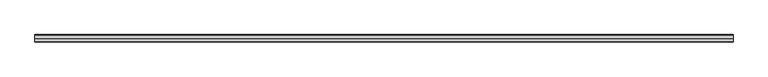
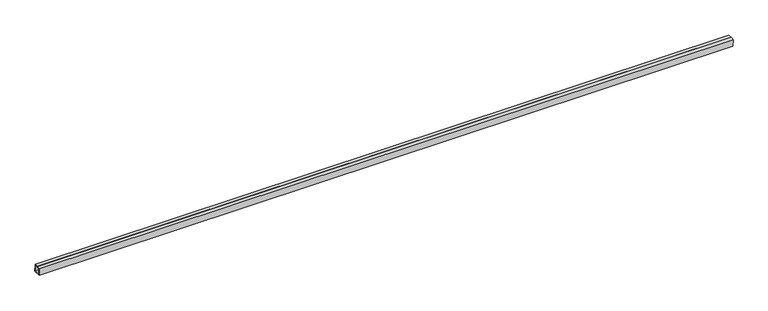
"""IFC4 building model written with IfcOpenShell, lengths in millimetres: proxy geometry, Inner panel:Inner panel:1:Inner panel:1 : Inner panel:Inner panel:300324:2:Inner panel:1:Inner panel:1 : Inner panel:Inner panel:300324:2 : Inner panel:Inner panel:1:Inner panel:1 : Inner panel:Inner panel:300324:300043:23 : Inner panel:Inner panel:1:Inner panel:1 : Inner panel:Inner panel:300324:2:Inner panel:1:Inner panel:1 : Inner panel:Inner panel:300324:2 : Inner panel:Inner panel:1:Inner panel:1 : Inner panel:Inner panel:300324:300043:308120."""

import ifcopenshell
import ifcopenshell.guid

model = None  # the IFC model being written
_history = None  # IfcOwnerHistory: only IFC2X3 demands one
_inside = {}  # id of a spatial element -> (the spatial element, [elements in it])
_under = {}  # id of a project, library or spatial element -> (it, [spatial elements below it])
_declared = {}  # id of a project -> (the project, [libraries it declares])
_typed = {}  # id of a type object -> (the type object, [elements of that type])
_made_of = {}  # id of a material, layer set ... -> (it, [elements and type objects made of it])


def new_model(schema):
    """Start an empty IFC model of exactly this schema.

    Asked for "IFC4X3", IfcOpenShell would pick the latest addendum, in which some entities
    have other attributes; the version numbers below select the first issue.
    IFC2X3 requires an IfcOwnerHistory on every rooted entity: one is made here for all.
    """
    global model, _history
    if schema == "IFC4X3":
        model = ifcopenshell.file(schema_version=(4, 3, 0, 0))
    else:
        model = ifcopenshell.file(schema=schema)
    _inside.clear()
    _under.clear()
    _declared.clear()
    _typed.clear()
    _made_of.clear()
    _history = None
    if model.schema == "IFC2X3":
        org = make("IfcOrganization", Name="unknown")
        user = make(
            "IfcPersonAndOrganization",
            ThePerson=make("IfcPerson", FamilyName="unknown"),
            TheOrganization=org,
        )
        app = make(
            "IfcApplication",
            ApplicationDeveloper=org,
            Version="unknown",
            ApplicationFullName="unknown",
            ApplicationIdentifier="unknown",
        )
        _history = make(
            "IfcOwnerHistory",
            OwningUser=user,
            OwningApplication=app,
            ChangeAction="ADDED",
            CreationDate=0,
        )
    return model


def make(cls, **values):
    """One entity of the class cls with the attributes given. An attribute that is None is left unset."""
    return model.create_entity(
        cls, **{name: value for name, value in values.items() if value is not None}
    )


def rooted(cls, **values):
    """An entity with a GlobalId (a new one), such as an element, a storey or a relation."""
    return make(cls, GlobalId=ifcopenshell.guid.new(), OwnerHistory=_history, **values)


def si_unit(unit_type, name, prefix=None):
    """IfcSIUnit, for example si_unit("LENGTHUNIT", "METRE", prefix="MILLI")."""
    return make("IfcSIUnit", UnitType=unit_type, Prefix=prefix, Name=name)


def assignment(units):
    """IfcUnitAssignment: the units of a project."""
    return None if units is None else make("IfcUnitAssignment", Units=units)


def point(xyz):
    """IfcCartesianPoint."""
    return None if xyz is None else make("IfcCartesianPoint", Coordinates=xyz)


def direction(xyz):
    """IfcDirection."""
    return None if xyz is None else make("IfcDirection", DirectionRatios=xyz)


def frame(location, z_axis=None, x_axis=None):
    """IfcAxis2Placement3D, a coordinate frame: its origin and axes. An axis left out is left unset."""
    return make(
        "IfcAxis2Placement3D",
        Location=point(location),
        Axis=direction(z_axis),
        RefDirection=direction(x_axis),
    )


def origin():
    """The frame at (0, 0, 0) with its axes left unset."""
    return frame((0.0, 0.0, 0.0))


def place(relative_to, where):
    """IfcLocalPlacement: puts the frame where relative to a parent placement (None: the world)."""
    return make(
        "IfcLocalPlacement", PlacementRelTo=relative_to, RelativePlacement=where
    )


def context(
    kind, dimensions, precision=None, world=None, true_north=None, identifier=None
):
    """IfcGeometricRepresentationContext, for example the 3D "Model" context."""
    return make(
        "IfcGeometricRepresentationContext",
        ContextIdentifier=identifier,
        ContextType=kind,
        CoordinateSpaceDimension=dimensions,
        Precision=precision,
        WorldCoordinateSystem=world,
        TrueNorth=true_north,
    )


def project(units=None, contexts=None):
    """IfcProject with its units and contexts."""
    return rooted(
        "IfcProject",
        Name="project",
        RepresentationContexts=contexts,
        UnitsInContext=assignment(units),
    )


def spatial(cls, under=None, at=None, **own):
    """A site, building, storey or space (cls), placed at a placement, below another one or the project."""
    s = rooted(cls, ObjectPlacement=at, **own)
    if under is not None:
        _under.setdefault(under.id(), (under, []))[1].append(s)
    return s


def polyline(points):
    """IfcPolyline through the points."""
    return make("IfcPolyline", Points=[point(p) for p in points])


def outline(outer, holes=None, kind="AREA"):
    """IfcArbitraryClosedProfileDef: a profile drawn as a closed curve; with holes, ...WithVoids."""
    if holes is None:
        return make("IfcArbitraryClosedProfileDef", ProfileType=kind, OuterCurve=outer)
    return make(
        "IfcArbitraryProfileDefWithVoids",
        ProfileType=kind,
        OuterCurve=outer,
        InnerCurves=holes,
    )


def extrude(swept, where, along, depth):
    """IfcExtrudedAreaSolid: the profile swept, set in the frame where, extruded along a direction by depth."""
    return make(
        "IfcExtrudedAreaSolid",
        SweptArea=swept,
        Position=where,
        ExtrudedDirection=direction(along),
        Depth=depth,
    )


def shape(context_of_items, identifier, shape_type, items):
    """IfcShapeRepresentation: the items that make up one representation, for example the "Body"."""
    return make(
        "IfcShapeRepresentation",
        ContextOfItems=context_of_items,
        RepresentationIdentifier=identifier,
        RepresentationType=shape_type,
        Items=items,
    )


def source(mapping_origin, context_of_items, identifier, shape_type, items):
    """IfcRepresentationMap: a shape defined once, which mapped items show again and again."""
    return make(
        "IfcRepresentationMap",
        MappingOrigin=mapping_origin,
        MappedRepresentation=shape(context_of_items, identifier, shape_type, items),
    )


def transform(
    local_origin,
    x_axis=None,
    y_axis=None,
    z_axis=None,
    scale=None,
    scale2=None,
    scale3=None,
    uniform=True,
):
    """IfcCartesianTransformationOperator3D, or its non-uniform kind. x_axis, y_axis, z_axis: its Axis1, 2, 3."""
    if uniform:
        return make(
            "IfcCartesianTransformationOperator3D",
            Axis1=direction(x_axis),
            Axis2=direction(y_axis),
            LocalOrigin=point(local_origin),
            Scale=scale,
            Axis3=direction(z_axis),
        )
    return make(
        "IfcCartesianTransformationOperator3DnonUniform",
        Axis1=direction(x_axis),
        Axis2=direction(y_axis),
        LocalOrigin=point(local_origin),
        Scale=scale,
        Axis3=direction(z_axis),
        Scale2=scale2,
        Scale3=scale3,
    )


def mapped(mapping_source, mapping_target):
    """IfcMappedItem: shows the shape of a source again, moved by a transform."""
    return make(
        "IfcMappedItem", MappingSource=mapping_source, MappingTarget=mapping_target
    )


def made_of(thing, what):
    """Note that an element or type object is made of a material, layer set ...; save() writes the relation."""
    if what is not None:
        _made_of.setdefault(what.id(), (what, []))[1].append(thing)
    return thing


def element(
    cls,
    number,
    at=None,
    inside=None,
    cuts=None,
    type_object=None,
    material=None,
    context=None,
    identifier="Body",
    shape_type=None,
    held_by="IfcProductDefinitionShape",
    body=None,
    shapes=None,
    **own,
):
    """One element of the class cls, such as IfcWall. Its Tag is "e" and its number.

    at: its placement. inside: the storey or other place that contains it. cuts: it is an
    opening in that element (IfcRelVoidsElement). A single representation is given by context,
    identifier, shape_type and body (its items); several are given by shapes. held_by: the class
    of the entity that holds the representations. save() writes the other relations.
    """
    e = rooted(cls, Tag="e%d" % number, ObjectPlacement=at, **own)
    if body is not None:
        shapes = [shape(context, identifier, shape_type, body)]
    if shapes is not None:
        e.Representation = make(held_by, Representations=shapes)
    if inside is not None:
        _inside.setdefault(inside.id(), (inside, []))[1].append(e)
    if cuts is not None:
        rooted(
            "IfcRelVoidsElement", RelatingBuildingElement=cuts, RelatedOpeningElement=e
        )
    if type_object is not None:
        _typed.setdefault(type_object.id(), (type_object, []))[1].append(e)
    return made_of(e, material)


def aggregate(whole, parts):
    """IfcRelAggregates: a whole, such as a stair, and the parts it consists of."""
    return rooted("IfcRelAggregates", RelatingObject=whole, RelatedObjects=parts)


def save(model, path):
    """Write the relations noted so far, then the file.

    IfcRelAggregates (storeys below a building ...), IfcRelContainedInSpatialStructure (elements
    in a storey), IfcRelDefinesByType, IfcRelAssociatesMaterial and IfcRelDeclares: one each for
    every whole, place, type object, material and project.
    """
    for whole, parts in _under.values():
        aggregate(whole, parts)
    for where, things in _inside.values():
        rooted(
            "IfcRelContainedInSpatialStructure",
            RelatedElements=things,
            RelatingStructure=where,
        )
    for kind, things in _typed.values():
        rooted("IfcRelDefinesByType", RelatedObjects=things, RelatingType=kind)
    for what, things in _made_of.values():
        rooted("IfcRelAssociatesMaterial", RelatedObjects=things, RelatingMaterial=what)
    for by, libraries in _declared.values():
        rooted("IfcRelDeclares", RelatingContext=by, RelatedDefinitions=libraries)
    model.write(path)


def generic_models_2387b0a6(model_context):
    return source(origin(), model_context, "Body", "SweptSolid", [
        extrude(outline(polyline([(-567056.8153809, 8850.7720379), (-567038.5749577, 8851.5320556), (-567036.988834, 8813.4650855), (-567075.0558041, 8811.8789617), (-567076.6419278, 8849.9459318), (-567058.4015047, 8850.7059494), (-567058.3023719, 8848.3267638), (-567074.1636095, 8847.6658789), (-567072.7757512, 8814.3572801), (-567039.4671523, 8815.7451384), (-567040.8550106, 8849.0537372), (-567056.7162482, 8848.3928523), (-567056.8153809, 8850.7720379)])), frame((593141.1867242, 0.0, 0.0), z_axis=(1.0, 0.0, 0.0), x_axis=(0.0, 1.0, 0.0)), (0.0, 0.0, 1.0), 3657.6),
    ])


if __name__ == "__main__":
    model = new_model("IFC4")
    model_context = context("Model", 3, world=origin())
    ifc_project = project(units=[si_unit("LENGTHUNIT", "METRE", prefix="MILLI")], contexts=[model_context])
    site = spatial("IfcSite", under=ifc_project)
    building = spatial("IfcBuilding", under=site)
    placement = place(None, origin())
    generic_models_shape = generic_models_2387b0a6(model_context)
    element("IfcBuildingElementProxy", 1, Name="Inner panel:Inner panel:1:Inner panel:1 : Inner panel:Inner panel:300324:2:Inner panel:1:Inner panel:1 : Inner panel:Inner panel:300324:2 : Inner panel:Inner panel:1:Inner panel:1 : Inner panel:Inner panel:300324:300043:23 : Inner panel:Inner panel:1:Inner panel:1 : Inner panel:Inner panel:300324:2:Inner panel:1:Inner panel:1 : Inner panel:Inner panel:300324:2 : Inner panel:Inner panel:1:Inner panel:1 : Inner panel:Inner panel:300324:300043:308120", ObjectType="Inner panel:Inner panel:1:Inner panel:1 : Inner panel:Inner panel:300324:2:Inner panel:1:Inner panel:1 : Inner panel:Inner panel:300324:2 : Inner panel:Inner panel:1:Inner panel:1 : Inner panel:Inner panel:300324:300043:23 : Inner panel:Inner panel:1:Inner panel:1 : Inner panel:Inner panel:300324:2:Inner panel:1:Inner panel:1 : Inner panel:Inner panel:300324:2 : Inner panel:Inner panel:1:Inner panel:1 : Inner panel:Inner panel:300324:300043:308120", at=placement, inside=building, context=model_context, shape_type="MappedRepresentation", body=[
        mapped(generic_models_shape, transform((0.0, 0.0, 0.0), x_axis=(1.0, 0.0, 0.0), y_axis=(0.0, 1.0, 0.0), z_axis=(0.0, 0.0, 1.0))),
    ])
    save(model, "model.ifc")

# Revit data of these elements
# Type "Inner panel:Inner panel:1:Inner panel:1 : Inner panel:Inner panel:300324:2:Inner panel:1:Inner panel:1 : Inner panel:Inner panel:300324:2 : Inner panel:Inner panel:1:Inner panel:1 : Inner panel:Inner panel:300324:300043:23 : Inner panel:Inner panel:1:Inner panel:1 : Inner panel:Inner panel:300324:2:Inner panel:1:Inner panel:1 : Inner panel:Inner panel:300324:2 : Inner panel:Inner panel:1:Inner panel:1 : Inner panel:Inner panel:300324:300043:308120"
#   NameOverride = "Inner panel:Inner panel:1:Inner panel:1 : Inner panel:Inner panel:300324:2:Inner panel:1:Inner panel:1 : Inner panel:Inner panel:300324:2 : Inner panel:Inner panel:1:Inner panel:1 : Inner panel:Inner panel:300324:300043:308120"
#   ObjectTypeOverride = "Inner panel:1:Inner panel:1 : Inner panel:Inner panel:300324:2 : Inner panel:Inner panel:1:Inner panel:1 : Inner panel:Inner panel:300324:300043"
#   Reference = "Inner panel"
#   Tag = "308120"
# Element 1 (IfcBuildingElementProxy, "Inner panel:Inner panel:1:Inner panel:1 : Inner panel:Inner panel:300324:2:Inner panel:1:Inner panel:1 : Inner panel:Inner panel:300324:2 : Inner panel:Inner panel:1:Inner panel:1 : Inner panel:Inner panel:300324:300043:23 : Inner panel:Inner panel:1:Inner panel:1 : Inner panel:Inner panel:300324:2:Inner panel:1:Inner panel:1 : Inner panel:Inner panel:300324:2 : Inner panel:Inner panel:1:Inner panel:1 : Inner panel:Inner panel:300324:300043:308120")
#   Materials on its faces: "1 1/2\" X 1 1/2\" SPLIT-SEAM SQUARE TUBING (~24\" CANTILEVER FROM C.L. OF GLULAM)"
# Materials
#   "1 1/2\" X 1 1/2\" SPLIT-SEAM SQUARE TUBING (~24\" CANTILEVER FROM C.L. OF GLULAM)": class "Unassigned", colour RGB 202 201 200, transparency 0, Cost = 0
